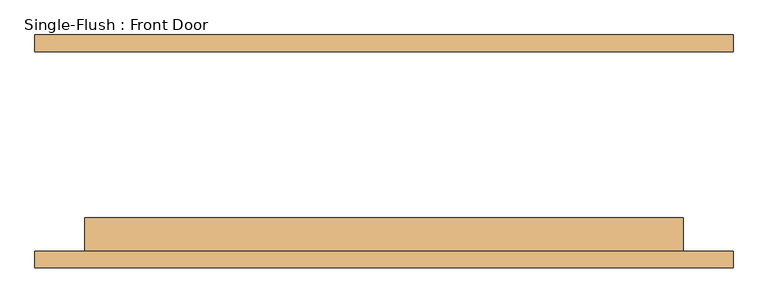
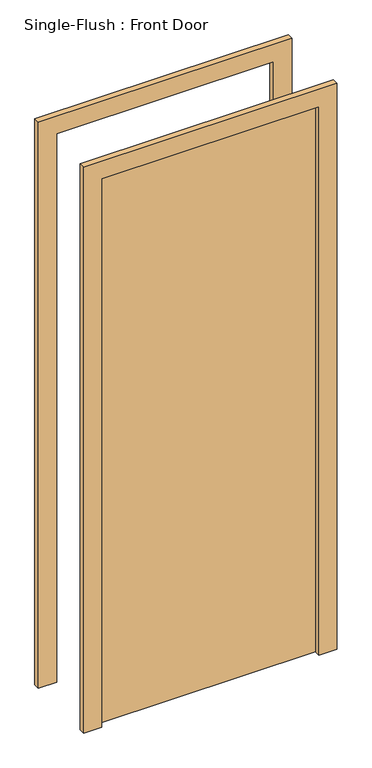
"""IFC4 building model written with IfcOpenShell, lengths in millimetres: door geometry, Single-Flush : Front Door."""

from ifc_helpers import new_model, si_unit, frame, origin, origin_with_axes, place, context, project, spatial, polyline, outline, extrude, source, transform, mapped, element, save


def single_flush_front_door_b84d2d09(model_context):
    return source(origin(), model_context, "Body", "SweptSolid", [
        extrude(outline(polyline([(2514.6, -533.4), (0.0, -533.4), (0.0, -457.2), (2438.4, -457.2), (2438.4, 457.2), (0.0, 457.2), (0.0, 533.4), (2514.6, 533.4), (2514.6, -533.4)])), frame((0.0, -177.8, 0.0), z_axis=(0.0, 1.0, 0.0), x_axis=(0.0, 0.0, 1.0)), (0.0, 0.0, 1.0), 25.4),
        extrude(outline(polyline([(2514.6, 533.4), (2514.6, -533.4), (0.0, -533.4), (0.0, -457.2), (2438.4, -457.2), (2438.4, 457.2), (0.0, 457.2), (0.0, 533.4), (2514.6, 533.4)])), frame((0.0, 152.4, 0.0), z_axis=(0.0, 1.0, 0.0), x_axis=(0.0, 0.0, 1.0)), (0.0, 0.0, 1.0), 25.4),
        extrude(outline(polyline([(457.2, -101.6), (457.2, -152.4), (-457.2, -152.4), (-457.2, -101.6), (457.2, -101.6)])), origin_with_axes(), (0.0, 0.0, 1.0), 2438.4),
    ])


if __name__ == "__main__":
    model = new_model("IFC4")
    model_context = context("Model", 3, world=origin())
    ifc_project = project(units=[si_unit("LENGTHUNIT", "METRE", prefix="MILLI")], contexts=[model_context])
    site = spatial("IfcSite", under=ifc_project)
    building = spatial("IfcBuilding", under=site)
    placement = place(None, origin())
    single_flush_front_door_shape = single_flush_front_door_b84d2d09(model_context)
    element("IfcDoor", 1, ObjectType="Single-Flush : Front Door", at=placement, inside=building, context=model_context, shape_type="MappedRepresentation", body=[
        mapped(single_flush_front_door_shape, transform((0.0, 0.0, 0.0), x_axis=(1.0, 0.0, 0.0), y_axis=(0.0, 1.0, 0.0), z_axis=(0.0, 0.0, 1.0))),
    ])
    save(model, "model.ifc")

# Revit data of these elements
# Type "Single-Flush : Front Door"
#   Type Mark = "36"
#   Assembly Code = "C1020"
#   Thickness = 0' - 2"
#   Height = 8' - 0"
#   Trim Projection Ext = 0' - 1"
#   Trim Projection Int = 0' - 1"
#   Trim Width = 0' - 3"
#   Width = 3' - 0"
#   Function = 0
#   Door Material = Metal - Paint Finish - Ivory,Matte
#   Frame Material = Concrete - Cast-in-Place Concrete
#   Wall Closure = (empty or 0)
# Element 1 (IfcDoor, "Single-Flush : Front Door")
#   Materials on its faces: "Concrete - Cast-in-Place Concrete", "Metal - Paint Finish - Ivory,Matte"
# Materials
#   "Metal - Paint Finish - Ivory,Matte": class "Paint", colour RGB 216 216 204, transparency 0, Comments = "Rendering appearance not upgraded Rendering appearance not upgraded "
#   "Concrete - Cast-in-Place Concrete": class "Concrete", colour RGB 178 178 178, transparency 0, Comments = "Rendering appearance not upgraded Rendering appearance not upgraded ", Description = "Concrete"
